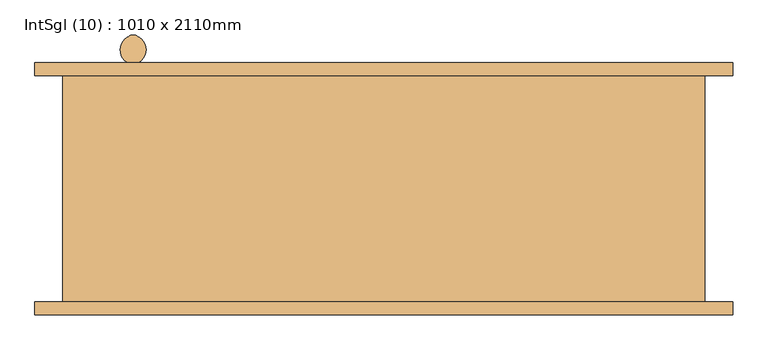
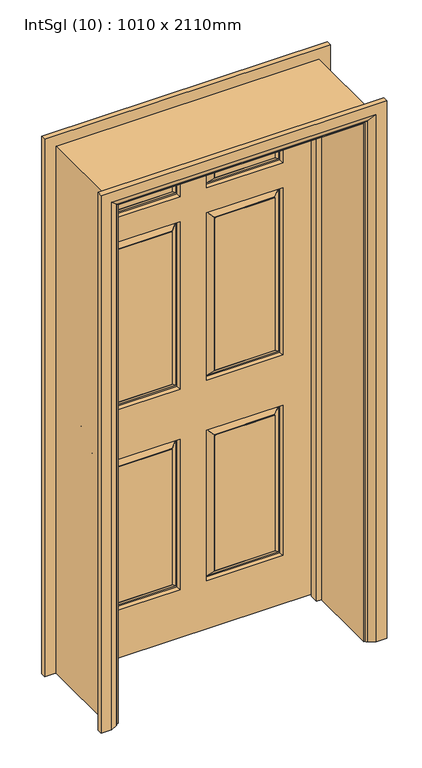
"""IFC4 building model written with IfcOpenShell, lengths in millimetres: door geometry, IntSgl (10) : 1010 x 2110mm."""

import ifcopenshell
import ifcopenshell.guid

model = None  # the IFC model being written
_history = None  # IfcOwnerHistory: only IFC2X3 demands one
_inside = {}  # id of a spatial element -> (the spatial element, [elements in it])
_under = {}  # id of a project, library or spatial element -> (it, [spatial elements below it])
_declared = {}  # id of a project -> (the project, [libraries it declares])
_typed = {}  # id of a type object -> (the type object, [elements of that type])
_made_of = {}  # id of a material, layer set ... -> (it, [elements and type objects made of it])


def new_model(schema):
    """Start an empty IFC model of exactly this schema.

    Asked for "IFC4X3", IfcOpenShell would pick the latest addendum, in which some entities
    have other attributes; the version numbers below select the first issue.
    IFC2X3 requires an IfcOwnerHistory on every rooted entity: one is made here for all.
    """
    global model, _history
    if schema == "IFC4X3":
        model = ifcopenshell.file(schema_version=(4, 3, 0, 0))
    else:
        model = ifcopenshell.file(schema=schema)
    _inside.clear()
    _under.clear()
    _declared.clear()
    _typed.clear()
    _made_of.clear()
    _history = None
    if model.schema == "IFC2X3":
        org = make("IfcOrganization", Name="unknown")
        user = make(
            "IfcPersonAndOrganization",
            ThePerson=make("IfcPerson", FamilyName="unknown"),
            TheOrganization=org,
        )
        app = make(
            "IfcApplication",
            ApplicationDeveloper=org,
            Version="unknown",
            ApplicationFullName="unknown",
            ApplicationIdentifier="unknown",
        )
        _history = make(
            "IfcOwnerHistory",
            OwningUser=user,
            OwningApplication=app,
            ChangeAction="ADDED",
            CreationDate=0,
        )
    return model


def make(cls, **values):
    """One entity of the class cls with the attributes given. An attribute that is None is left unset."""
    return model.create_entity(
        cls, **{name: value for name, value in values.items() if value is not None}
    )


def rooted(cls, **values):
    """An entity with a GlobalId (a new one), such as an element, a storey or a relation."""
    return make(cls, GlobalId=ifcopenshell.guid.new(), OwnerHistory=_history, **values)


def si_unit(unit_type, name, prefix=None):
    """IfcSIUnit, for example si_unit("LENGTHUNIT", "METRE", prefix="MILLI")."""
    return make("IfcSIUnit", UnitType=unit_type, Prefix=prefix, Name=name)


def assignment(units):
    """IfcUnitAssignment: the units of a project."""
    return None if units is None else make("IfcUnitAssignment", Units=units)


def point(xyz):
    """IfcCartesianPoint."""
    return None if xyz is None else make("IfcCartesianPoint", Coordinates=xyz)


def direction(xyz):
    """IfcDirection."""
    return None if xyz is None else make("IfcDirection", DirectionRatios=xyz)


def frame(location, z_axis=None, x_axis=None):
    """IfcAxis2Placement3D, a coordinate frame: its origin and axes. An axis left out is left unset."""
    return make(
        "IfcAxis2Placement3D",
        Location=point(location),
        Axis=direction(z_axis),
        RefDirection=direction(x_axis),
    )


def origin():
    """The frame at (0, 0, 0) with its axes left unset."""
    return frame((0.0, 0.0, 0.0))


def place(relative_to, where):
    """IfcLocalPlacement: puts the frame where relative to a parent placement (None: the world)."""
    return make(
        "IfcLocalPlacement", PlacementRelTo=relative_to, RelativePlacement=where
    )


def context(
    kind, dimensions, precision=None, world=None, true_north=None, identifier=None
):
    """IfcGeometricRepresentationContext, for example the 3D "Model" context."""
    return make(
        "IfcGeometricRepresentationContext",
        ContextIdentifier=identifier,
        ContextType=kind,
        CoordinateSpaceDimension=dimensions,
        Precision=precision,
        WorldCoordinateSystem=world,
        TrueNorth=true_north,
    )


def project(units=None, contexts=None):
    """IfcProject with its units and contexts."""
    return rooted(
        "IfcProject",
        Name="project",
        RepresentationContexts=contexts,
        UnitsInContext=assignment(units),
    )


def spatial(cls, under=None, at=None, **own):
    """A site, building, storey or space (cls), placed at a placement, below another one or the project."""
    s = rooted(cls, ObjectPlacement=at, **own)
    if under is not None:
        _under.setdefault(under.id(), (under, []))[1].append(s)
    return s


def polyline(points):
    """IfcPolyline through the points."""
    return make("IfcPolyline", Points=[point(p) for p in points])


def circle_curve(where, radius):
    """IfcCircle in the frame where."""
    return make("IfcCircle", Position=where, Radius=radius)


def ellipse_curve(where, semi_axis1, semi_axis2):
    """IfcEllipse in the frame where."""
    return make(
        "IfcEllipse", Position=where, SemiAxis1=semi_axis1, SemiAxis2=semi_axis2
    )


def trimmed(basis, trim1, trim2, sense, master):
    """IfcTrimmedCurve: the piece of a basis curve between two trims."""
    return make(
        "IfcTrimmedCurve",
        BasisCurve=basis,
        Trim1=trim1,
        Trim2=trim2,
        SenseAgreement=sense,
        MasterRepresentation=master,
    )


def outline(outer, holes=None, kind="AREA"):
    """IfcArbitraryClosedProfileDef: a profile drawn as a closed curve; with holes, ...WithVoids."""
    if holes is None:
        return make("IfcArbitraryClosedProfileDef", ProfileType=kind, OuterCurve=outer)
    return make(
        "IfcArbitraryProfileDefWithVoids",
        ProfileType=kind,
        OuterCurve=outer,
        InnerCurves=holes,
    )


def extrude(swept, where, along, depth):
    """IfcExtrudedAreaSolid: the profile swept, set in the frame where, extruded along a direction by depth."""
    return make(
        "IfcExtrudedAreaSolid",
        SweptArea=swept,
        Position=where,
        ExtrudedDirection=direction(along),
        Depth=depth,
    )


def faces_of(points, faces, orient=None, outer=None):
    """IfcFace entities. A face is a list of loops; a loop is a list of indices into points, from 0.

    orient and outer hold one flag for each loop. By default every Orientation is true, the
    first loop of a face is its IfcFaceOuterBound and the others are IfcFaceBound.
    """
    made = []
    for i, loops in enumerate(faces):
        bounds = []
        for j, loop in enumerate(loops):
            is_outer = j == 0 if outer is None else outer[i][j]
            bounds.append(
                make(
                    "IfcFaceOuterBound" if is_outer else "IfcFaceBound",
                    Bound=make("IfcPolyLoop", Polygon=[points[k] for k in loop]),
                    Orientation=True if orient is None else orient[i][j],
                )
            )
        made.append(make("IfcFace", Bounds=bounds))
    return made


def faceted_brep(points, faces, orient=None, outer=None, voids=None):
    """IfcFacetedBrep: a solid bounded by flat faces; with voids (closed shells), ...WithVoids."""
    shared = [point(p) for p in points]
    hull = make("IfcClosedShell", CfsFaces=faces_of(shared, faces, orient, outer))
    if voids is None:
        return make("IfcFacetedBrep", Outer=hull)
    return make(
        "IfcFacetedBrepWithVoids",
        Outer=hull,
        Voids=[
            make(cls, CfsFaces=faces_of(shared, fs, o, b)) for cls, fs, o, b in voids
        ],
    )


def shape(context_of_items, identifier, shape_type, items):
    """IfcShapeRepresentation: the items that make up one representation, for example the "Body"."""
    return make(
        "IfcShapeRepresentation",
        ContextOfItems=context_of_items,
        RepresentationIdentifier=identifier,
        RepresentationType=shape_type,
        Items=items,
    )


def source(mapping_origin, context_of_items, identifier, shape_type, items):
    """IfcRepresentationMap: a shape defined once, which mapped items show again and again."""
    return make(
        "IfcRepresentationMap",
        MappingOrigin=mapping_origin,
        MappedRepresentation=shape(context_of_items, identifier, shape_type, items),
    )


def transform(
    local_origin,
    x_axis=None,
    y_axis=None,
    z_axis=None,
    scale=None,
    scale2=None,
    scale3=None,
    uniform=True,
):
    """IfcCartesianTransformationOperator3D, or its non-uniform kind. x_axis, y_axis, z_axis: its Axis1, 2, 3."""
    if uniform:
        return make(
            "IfcCartesianTransformationOperator3D",
            Axis1=direction(x_axis),
            Axis2=direction(y_axis),
            LocalOrigin=point(local_origin),
            Scale=scale,
            Axis3=direction(z_axis),
        )
    return make(
        "IfcCartesianTransformationOperator3DnonUniform",
        Axis1=direction(x_axis),
        Axis2=direction(y_axis),
        LocalOrigin=point(local_origin),
        Scale=scale,
        Axis3=direction(z_axis),
        Scale2=scale2,
        Scale3=scale3,
    )


def mapped(mapping_source, mapping_target):
    """IfcMappedItem: shows the shape of a source again, moved by a transform."""
    return make(
        "IfcMappedItem", MappingSource=mapping_source, MappingTarget=mapping_target
    )


def made_of(thing, what):
    """Note that an element or type object is made of a material, layer set ...; save() writes the relation."""
    if what is not None:
        _made_of.setdefault(what.id(), (what, []))[1].append(thing)
    return thing


def element(
    cls,
    number,
    at=None,
    inside=None,
    cuts=None,
    type_object=None,
    material=None,
    context=None,
    identifier="Body",
    shape_type=None,
    held_by="IfcProductDefinitionShape",
    body=None,
    shapes=None,
    **own,
):
    """One element of the class cls, such as IfcWall. Its Tag is "e" and its number.

    at: its placement. inside: the storey or other place that contains it. cuts: it is an
    opening in that element (IfcRelVoidsElement). A single representation is given by context,
    identifier, shape_type and body (its items); several are given by shapes. held_by: the class
    of the entity that holds the representations. save() writes the other relations.
    """
    e = rooted(cls, Tag="e%d" % number, ObjectPlacement=at, **own)
    if body is not None:
        shapes = [shape(context, identifier, shape_type, body)]
    if shapes is not None:
        e.Representation = make(held_by, Representations=shapes)
    if inside is not None:
        _inside.setdefault(inside.id(), (inside, []))[1].append(e)
    if cuts is not None:
        rooted(
            "IfcRelVoidsElement", RelatingBuildingElement=cuts, RelatedOpeningElement=e
        )
    if type_object is not None:
        _typed.setdefault(type_object.id(), (type_object, []))[1].append(e)
    return made_of(e, material)


def aggregate(whole, parts):
    """IfcRelAggregates: a whole, such as a stair, and the parts it consists of."""
    return rooted("IfcRelAggregates", RelatingObject=whole, RelatedObjects=parts)


def save(model, path):
    """Write the relations noted so far, then the file.

    IfcRelAggregates (storeys below a building ...), IfcRelContainedInSpatialStructure (elements
    in a storey), IfcRelDefinesByType, IfcRelAssociatesMaterial and IfcRelDeclares: one each for
    every whole, place, type object, material and project.
    """
    for whole, parts in _under.values():
        aggregate(whole, parts)
    for where, things in _inside.values():
        rooted(
            "IfcRelContainedInSpatialStructure",
            RelatedElements=things,
            RelatingStructure=where,
        )
    for kind, things in _typed.values():
        rooted("IfcRelDefinesByType", RelatedObjects=things, RelatingType=kind)
    for what, things in _made_of.values():
        rooted("IfcRelAssociatesMaterial", RelatedObjects=things, RelatingMaterial=what)
    for by, libraries in _declared.values():
        rooted("IfcRelDeclares", RelatingContext=by, RelatedDefinitions=libraries)
    model.write(path)


def plane_surface(at):
    """IfcPlane: the flat surface through the origin of the frame at, square to its z axis."""
    return make("IfcPlane", Position=at)


def cylinder_surface(at, radius):
    """IfcCylindricalSurface: all points at the distance radius from the z axis of the frame at."""
    return make("IfcCylindricalSurface", Position=at, Radius=radius)


def revolved_surface(curve, axis_point, axis_direction):
    """IfcSurfaceOfRevolution: the curve turned about the line through axis_point along axis_direction."""
    return make(
        "IfcSurfaceOfRevolution",
        SweptCurve=make("IfcArbitraryOpenProfileDef", ProfileType="CURVE", Curve=curve),
        AxisPosition=make("IfcAxis1Placement", Location=point(axis_point), Axis=direction(axis_direction)),
    )


def advanced_brep(points, edges, surfaces, faces):
    """IfcAdvancedBrep: a solid bounded by faces that lie on surfaces and meet in shared edges.

    An edge is (start, end): straight between two places in points (the first is 0);
    or (start, end, curve); or (start, end, curve, False) where it runs against its curve.
    A face is (place in surfaces, loops), or (place, loops, False) where it looks against
    its surface's normal. A loop lists edges by number (the first is 1), with a minus sign
    where the edge is run from its end to its start. The first loop is the outer one.
    """
    corners = [point(p) for p in points]
    vertices = [make("IfcVertexPoint", VertexGeometry=c) for c in corners]
    made = []
    for start, end, *more in edges:
        made.append(
            make(
                "IfcEdgeCurve",
                EdgeStart=vertices[start],
                EdgeEnd=vertices[end],
                EdgeGeometry=more[0] if more else make("IfcPolyline", Points=[corners[start], corners[end]]),
                SameSense=more[1] if len(more) > 1 else True,
            )
        )
    hull = []
    for where, loops, *sense in faces:
        bounds = []
        for j, loop in enumerate(loops):
            ring = [make("IfcOrientedEdge", EdgeElement=made[abs(k) - 1], Orientation=k > 0) for k in loop]
            bounds.append(
                make(
                    "IfcFaceOuterBound" if j == 0 else "IfcFaceBound",
                    Bound=make("IfcEdgeLoop", EdgeList=ring),
                    Orientation=True,
                )
            )
        hull.append(make("IfcAdvancedFace", Bounds=bounds, FaceSurface=surfaces[where], SameSense=sense[0] if sense else True))
    return make("IfcAdvancedBrep", Outer=make("IfcClosedShell", CfsFaces=hull))


def intsgl_10_1010_x_2110mm_e5549126(model_context):
    return source(origin(), model_context, "Body", "SolidModel", [
        advanced_brep(
        [(-383.0, 118.0, 900.0), (-388.0, 73.562589, 900.0), (-393.0, 118.0, 900.0), (-393.0, 133.0, 900.0), (-383.0, 133.0, 900.0), (-408.0, 137.0, 900.0), (-368.0, 137.0, 900.0), (-408.0, 133.0, 900.0), (-368.0, 133.0, 900.0)],
        [
            (0, 1, circle_curve(frame((-391.1884862, 96.4213505, 900.0), z_axis=(0.0, 0.0, -1.0), x_axis=(0.0, 1.0, 0.0)), 23.0800654)),
            (1, 2, circle_curve(frame((-384.8115138, 96.4213505, 900.0), z_axis=(0.0, 0.0, -1.0), x_axis=(0.0, 1.0, 0.0)), 23.0800654)),
            (2, 0, circle_curve(frame((-388.0, 118.0, 900.0), z_axis=(0.0, -1.0, 0.0), x_axis=(-1.0, 0.0, 0.0)), 5.0)),
            (0, 2, circle_curve(frame((-388.0, 118.0, 900.0), z_axis=(0.0, -1.0, 0.0), x_axis=(-1.0, 0.0, 0.0)), 5.0)),
            (2, 3),
            (3, 4, circle_curve(frame((-388.0, 133.0, 900.0), z_axis=(0.0, -1.0, 0.0), x_axis=(-1.0, 0.0, 0.0)), 5.0)),
            (4, 0),
            (4, 3, circle_curve(frame((-388.0, 133.0, 900.0), z_axis=(0.0, -1.0, 0.0), x_axis=(-1.0, 0.0, 0.0)), 5.0)),
            (5, 6, circle_curve(frame((-388.0, 137.0, 900.0), z_axis=(0.0, 1.0, 0.0), x_axis=(1.0, 0.0, 0.0)), 20.0)),
            (6, 5, circle_curve(frame((-388.0, 137.0, 900.0), z_axis=(0.0, 1.0, 0.0), x_axis=(1.0, 0.0, 0.0)), 20.0)),
            (7, 8, circle_curve(frame((-388.0, 133.0, 900.0), z_axis=(0.0, -1.0, 0.0), x_axis=(1.0, 0.0, 0.0)), 20.0)),
            (8, 7, circle_curve(frame((-388.0, 133.0, 900.0), z_axis=(0.0, -1.0, 0.0), x_axis=(1.0, 0.0, 0.0)), 20.0)),
            (6, 8),
            (7, 5),
        ],
        [
            revolved_surface(trimmed(ellipse_curve(frame((-384.8115138, 96.4213505, 900.0), z_axis=(0.0, 0.0, -1.0), x_axis=(0.0, 1.0, 0.0)), 23.0800654, 23.0800654), [point((-388.0, 73.562589, 900.0))], [point((-393.0, 118.0, 900.0))], True, "CARTESIAN"), (-388.0, 133.0, 900.0), (0.0, 1.0, 0.0)),
            cylinder_surface(frame((-388.0, 133.0, 900.0), z_axis=(0.0, 1.0, 0.0), x_axis=(-1.0, 0.0, 0.0)), 5.0),
            plane_surface(frame((-368.0, 137.0, 900.0), z_axis=(0.0, 1.0, 0.0), x_axis=(0.0, 0.0, 1.0))),
            plane_surface(frame((-368.0, 133.0, 900.0), z_axis=(0.0, -1.0, 0.0), x_axis=(0.0, 0.0, -1.0))),
            cylinder_surface(frame((-388.0, 133.0, 900.0), z_axis=(0.0, 1.0, 0.0), x_axis=(1.0, 0.0, 0.0)), 20.0),
        ],
        [
            (0, [[1, 2, 3]]),
            (0, [[-1, 4, -2]]),
            (1, [[5, 6, 7, -3]]),
            (1, [[-7, 8, -5, -4]]),
            (2, [[9, 10]]),
            (3, [[11, 12], [-8, -6]]),
            (4, [[13, -11, 14, -10]]),
            (4, [[-14, -12, -13, -9]]),
        ],
    ),
        advanced_brep(
        [(-383.0, 194.0, 900.0), (-393.0, 194.0, 900.0), (-388.0, 238.437411, 900.0), (-383.0, 179.0, 900.0), (-393.0, 179.0, 900.0), (-408.0, 175.0, 900.0), (-368.0, 175.0, 900.0), (-408.0, 179.0, 900.0), (-368.0, 179.0, 900.0)],
        [
            (0, 1, circle_curve(frame((-388.0, 194.0, 900.0), z_axis=(0.0, 1.0, 0.0), x_axis=(-1.0, 0.0, 0.0)), 5.0)),
            (1, 2, circle_curve(frame((-384.8115138, 215.5786495, 900.0), z_axis=(0.0, 0.0, -1.0), x_axis=(0.0, -1.0, 0.0)), 23.0800654)),
            (2, 0, circle_curve(frame((-391.1884862, 215.5786495, 900.0), z_axis=(0.0, 0.0, -1.0), x_axis=(0.0, -1.0, 0.0)), 23.0800654)),
            (1, 0, circle_curve(frame((-388.0, 194.0, 900.0), z_axis=(0.0, 1.0, 0.0), x_axis=(-1.0, 0.0, 0.0)), 5.0)),
            (0, 3),
            (3, 4, circle_curve(frame((-388.0, 179.0, 900.0), z_axis=(0.0, 1.0, 0.0), x_axis=(-1.0, 0.0, 0.0)), 5.0)),
            (4, 1),
            (4, 3, circle_curve(frame((-388.0, 179.0, 900.0), z_axis=(0.0, 1.0, 0.0), x_axis=(-1.0, 0.0, 0.0)), 5.0)),
            (5, 6, circle_curve(frame((-388.0, 175.0, 900.0), z_axis=(0.0, -1.0, 0.0), x_axis=(1.0, 0.0, 0.0)), 20.0)),
            (6, 5, circle_curve(frame((-388.0, 175.0, 900.0), z_axis=(0.0, -1.0, 0.0), x_axis=(1.0, 0.0, 0.0)), 20.0)),
            (7, 8, circle_curve(frame((-388.0, 179.0, 900.0), z_axis=(0.0, 1.0, 0.0), x_axis=(1.0, 0.0, 0.0)), 20.0)),
            (8, 7, circle_curve(frame((-388.0, 179.0, 900.0), z_axis=(0.0, 1.0, 0.0), x_axis=(1.0, 0.0, 0.0)), 20.0)),
            (5, 7),
            (8, 6),
        ],
        [
            revolved_surface(trimmed(ellipse_curve(frame((-384.8115138, 215.5786495, 900.0), z_axis=(0.0, 0.0, 1.0), x_axis=(0.0, -1.0, 0.0)), 23.0800654, 23.0800654), [point((-388.0, 238.437411, 900.0))], [point((-393.0, 194.0, 900.0))], True, "CARTESIAN"), (-388.0, 179.0, 900.0), (0.0, -1.0, 0.0)),
            cylinder_surface(frame((-388.0, 179.0, 900.0), z_axis=(0.0, -1.0, 0.0), x_axis=(-1.0, 0.0, 0.0)), 5.0),
            plane_surface(frame((-368.0, 175.0, 900.0), z_axis=(0.0, -1.0, 0.0), x_axis=(0.0, 0.0, 1.0))),
            plane_surface(frame((-368.0, 179.0, 900.0), z_axis=(0.0, 1.0, 0.0), x_axis=(0.0, 0.0, -1.0))),
            cylinder_surface(frame((-388.0, 179.0, 900.0), z_axis=(0.0, -1.0, 0.0), x_axis=(1.0, 0.0, 0.0)), 20.0),
        ],
        [
            (0, [[1, 2, 3]]),
            (0, [[-2, 4, -3]]),
            (1, [[-1, 5, 6, 7]]),
            (1, [[-4, -7, 8, -5]]),
            (2, [[9, 10]]),
            (3, [[11, 12], [-6, -8]]),
            (4, [[-9, 13, -12, 14]]),
            (4, [[-10, -14, -11, -13]]),
        ],
    ),
        faceted_brep([(-463.0, 137.0, 2068.0), (-463.0, 137.0, 8.0), (463.0, 137.0, 8.0), (463.0, 137.0, 2068.0), (-50.0, 137.0, 800.0), (-50.0, 137.0, 200.0), (-338.0, 137.0, 200.0), (-338.0, 137.0, 800.0), (338.0, 137.0, 800.0), (338.0, 137.0, 200.0), (50.0, 137.0, 200.0), (50.0, 137.0, 800.0), (-50.0, 137.0, 1668.0), (-50.0, 137.0, 1000.0), (-338.0, 137.0, 1000.0), (-338.0, 137.0, 1668.0), (338.0, 137.0, 1668.0), (338.0, 137.0, 1000.0), (50.0, 137.0, 1000.0), (50.0, 137.0, 1668.0), (-50.0, 137.0, 1943.0), (-50.0, 137.0, 1768.0), (-338.0, 137.0, 1768.0), (-338.0, 137.0, 1943.0), (338.0, 137.0, 1943.0), (338.0, 137.0, 1768.0), (50.0, 137.0, 1768.0), (50.0, 137.0, 1943.0), (-80.0, 137.0, 230.0), (-80.0, 137.0, 770.0), (-308.0, 137.0, 770.0), (-308.0, 137.0, 230.0), (308.0, 137.0, 230.0), (308.0, 137.0, 770.0), (80.0, 137.0, 770.0), (80.0, 137.0, 230.0), (-80.0, 137.0, 1030.0), (-80.0, 137.0, 1638.0), (-308.0, 137.0, 1638.0), (-308.0, 137.0, 1030.0), (308.0, 137.0, 1030.0), (308.0, 137.0, 1638.0), (80.0, 137.0, 1638.0), (80.0, 137.0, 1030.0), (-80.0, 137.0, 1798.0), (-80.0, 137.0, 1913.0), (-308.0, 137.0, 1913.0), (-308.0, 137.0, 1798.0), (308.0, 137.0, 1798.0), (308.0, 137.0, 1913.0), (80.0, 137.0, 1913.0), (80.0, 137.0, 1798.0), (-463.0, 175.0, 2068.0), (463.0, 175.0, 2068.0), (463.0, 175.0, 8.0), (-463.0, 175.0, 8.0), (50.0, 175.0, 800.0), (50.0, 175.0, 200.0), (338.0, 175.0, 200.0), (338.0, 175.0, 800.0), (-338.0, 175.0, 800.0), (-338.0, 175.0, 200.0), (-50.0, 175.0, 200.0), (-50.0, 175.0, 800.0), (50.0, 175.0, 1668.0), (50.0, 175.0, 1000.0), (338.0, 175.0, 1000.0), (338.0, 175.0, 1668.0), (-338.0, 175.0, 1668.0), (-338.0, 175.0, 1000.0), (-50.0, 175.0, 1000.0), (-50.0, 175.0, 1668.0), (50.0, 175.0, 1943.0), (50.0, 175.0, 1768.0), (338.0, 175.0, 1768.0), (338.0, 175.0, 1943.0), (-338.0, 175.0, 1943.0), (-338.0, 175.0, 1768.0), (-50.0, 175.0, 1768.0), (-50.0, 175.0, 1943.0), (80.0, 175.0, 230.0), (80.0, 175.0, 770.0), (308.0, 175.0, 770.0), (308.0, 175.0, 230.0), (-308.0, 175.0, 230.0), (-308.0, 175.0, 770.0), (-80.0, 175.0, 770.0), (-80.0, 175.0, 230.0), (80.0, 175.0, 1030.0), (80.0, 175.0, 1638.0), (308.0, 175.0, 1638.0), (308.0, 175.0, 1030.0), (-308.0, 175.0, 1030.0), (-308.0, 175.0, 1638.0), (-80.0, 175.0, 1638.0), (-80.0, 175.0, 1030.0), (80.0, 175.0, 1798.0), (80.0, 175.0, 1913.0), (308.0, 175.0, 1913.0), (308.0, 175.0, 1798.0), (-308.0, 175.0, 1798.0), (-308.0, 175.0, 1913.0), (-80.0, 175.0, 1913.0), (-80.0, 175.0, 1798.0), (80.0, 174.0, 230.0), (80.0, 174.0, 770.0), (58.0, 160.0, 208.0), (58.0, 160.0, 792.0), (78.0, 174.0, 772.0), (78.0, 174.0, 228.0), (53.0, 160.0, 797.0), (53.0, 160.0, 203.0), (308.0, 174.0, 770.0), (330.0, 160.0, 792.0), (310.0, 174.0, 772.0), (335.0, 160.0, 797.0), (308.0, 174.0, 230.0), (330.0, 160.0, 208.0), (310.0, 174.0, 228.0), (335.0, 160.0, 203.0), (-308.0, 174.0, 230.0), (-308.0, 174.0, 770.0), (-330.0, 160.0, 208.0), (-330.0, 160.0, 792.0), (-310.0, 174.0, 772.0), (-310.0, 174.0, 228.0), (-335.0, 160.0, 797.0), (-335.0, 160.0, 203.0), (-80.0, 174.0, 770.0), (-58.0, 160.0, 792.0), (-78.0, 174.0, 772.0), (-53.0, 160.0, 797.0), (-80.0, 174.0, 230.0), (-58.0, 160.0, 208.0), (-78.0, 174.0, 228.0), (-53.0, 160.0, 203.0), (80.0, 174.0, 1030.0), (80.0, 174.0, 1638.0), (58.0, 160.0, 1008.0), (58.0, 160.0, 1660.0), (78.0, 174.0, 1640.0), (78.0, 174.0, 1028.0), (53.0, 160.0, 1665.0), (53.0, 160.0, 1003.0), (308.0, 174.0, 1638.0), (330.0, 160.0, 1660.0), (310.0, 174.0, 1640.0), (335.0, 160.0, 1665.0), (308.0, 174.0, 1030.0), (330.0, 160.0, 1008.0), (310.0, 174.0, 1028.0), (335.0, 160.0, 1003.0), (-308.0, 174.0, 1030.0), (-308.0, 174.0, 1638.0), (-330.0, 160.0, 1008.0), (-330.0, 160.0, 1660.0), (-310.0, 174.0, 1640.0), (-310.0, 174.0, 1028.0), (-335.0, 160.0, 1665.0), (-335.0, 160.0, 1003.0), (-80.0, 174.0, 1638.0), (-58.0, 160.0, 1660.0), (-78.0, 174.0, 1640.0), (-53.0, 160.0, 1665.0), (-80.0, 174.0, 1030.0), (-58.0, 160.0, 1008.0), (-78.0, 174.0, 1028.0), (-53.0, 160.0, 1003.0), (80.0, 174.0, 1798.0), (80.0, 174.0, 1913.0), (58.0, 160.0, 1776.0), (58.0, 160.0, 1935.0), (78.0, 174.0, 1915.0), (78.0, 174.0, 1796.0), (53.0, 160.0, 1940.0), (53.0, 160.0, 1771.0), (308.0, 174.0, 1913.0), (330.0, 160.0, 1935.0), (310.0, 174.0, 1915.0), (335.0, 160.0, 1940.0), (308.0, 174.0, 1798.0), (330.0, 160.0, 1776.0), (310.0, 174.0, 1796.0), (335.0, 160.0, 1771.0), (-308.0, 174.0, 1798.0), (-308.0, 174.0, 1913.0), (-330.0, 160.0, 1776.0), (-330.0, 160.0, 1935.0), (-310.0, 174.0, 1915.0), (-310.0, 174.0, 1796.0), (-335.0, 160.0, 1940.0), (-335.0, 160.0, 1771.0), (-80.0, 174.0, 1913.0), (-58.0, 160.0, 1935.0), (-78.0, 174.0, 1915.0), (-53.0, 160.0, 1940.0), (-80.0, 174.0, 1798.0), (-58.0, 160.0, 1776.0), (-78.0, 174.0, 1796.0), (-53.0, 160.0, 1771.0), (-80.0, 138.0, 230.0), (-80.0, 138.0, 770.0), (-58.0, 152.0, 208.0), (-58.0, 152.0, 792.0), (-78.0, 138.0, 772.0), (-78.0, 138.0, 228.0), (-53.0, 152.0, 797.0), (-53.0, 152.0, 203.0), (-308.0, 138.0, 770.0), (-330.0, 152.0, 792.0), (-310.0, 138.0, 772.0), (-335.0, 152.0, 797.0), (-308.0, 138.0, 230.0), (-330.0, 152.0, 208.0), (-310.0, 138.0, 228.0), (-335.0, 152.0, 203.0), (308.0, 138.0, 230.0), (308.0, 138.0, 770.0), (330.0, 152.0, 208.0), (330.0, 152.0, 792.0), (310.0, 138.0, 772.0), (310.0, 138.0, 228.0), (335.0, 152.0, 797.0), (335.0, 152.0, 203.0), (80.0, 138.0, 770.0), (58.0, 152.0, 792.0), (78.0, 138.0, 772.0), (53.0, 152.0, 797.0), (80.0, 138.0, 230.0), (58.0, 152.0, 208.0), (78.0, 138.0, 228.0), (53.0, 152.0, 203.0), (-80.0, 138.0, 1030.0), (-80.0, 138.0, 1638.0), (-58.0, 152.0, 1008.0), (-58.0, 152.0, 1660.0), (-78.0, 138.0, 1640.0), (-78.0, 138.0, 1028.0), (-53.0, 152.0, 1665.0), (-53.0, 152.0, 1003.0), (-308.0, 138.0, 1638.0), (-330.0, 152.0, 1660.0), (-310.0, 138.0, 1640.0), (-335.0, 152.0, 1665.0), (-308.0, 138.0, 1030.0), (-330.0, 152.0, 1008.0), (-310.0, 138.0, 1028.0), (-335.0, 152.0, 1003.0), (308.0, 138.0, 1030.0), (308.0, 138.0, 1638.0), (330.0, 152.0, 1008.0), (330.0, 152.0, 1660.0), (310.0, 138.0, 1640.0), (310.0, 138.0, 1028.0), (335.0, 152.0, 1665.0), (335.0, 152.0, 1003.0), (80.0, 138.0, 1638.0), (58.0, 152.0, 1660.0), (78.0, 138.0, 1640.0), (53.0, 152.0, 1665.0), (80.0, 138.0, 1030.0), (58.0, 152.0, 1008.0), (78.0, 138.0, 1028.0), (53.0, 152.0, 1003.0), (-80.0, 138.0, 1798.0), (-80.0, 138.0, 1913.0), (-58.0, 152.0, 1776.0), (-58.0, 152.0, 1935.0), (-78.0, 138.0, 1915.0), (-78.0, 138.0, 1796.0), (-53.0, 152.0, 1940.0), (-53.0, 152.0, 1771.0), (-308.0, 138.0, 1913.0), (-330.0, 152.0, 1935.0), (-310.0, 138.0, 1915.0), (-335.0, 152.0, 1940.0), (-308.0, 138.0, 1798.0), (-330.0, 152.0, 1776.0), (-310.0, 138.0, 1796.0), (-335.0, 152.0, 1771.0), (308.0, 138.0, 1798.0), (308.0, 138.0, 1913.0), (330.0, 152.0, 1776.0), (330.0, 152.0, 1935.0), (310.0, 138.0, 1915.0), (310.0, 138.0, 1796.0), (335.0, 152.0, 1940.0), (335.0, 152.0, 1771.0), (80.0, 138.0, 1913.0), (58.0, 152.0, 1935.0), (78.0, 138.0, 1915.0), (53.0, 152.0, 1940.0), (80.0, 138.0, 1798.0), (58.0, 152.0, 1776.0), (78.0, 138.0, 1796.0), (53.0, 152.0, 1771.0)], [[[0, 1, 2, 3], [4, 5, 6, 7], [8, 9, 10, 11], [12, 13, 14, 15], [16, 17, 18, 19], [20, 21, 22, 23], [24, 25, 26, 27]], [[28, 29, 30, 31]], [[32, 33, 34, 35]], [[36, 37, 38, 39]], [[40, 41, 42, 43]], [[44, 45, 46, 47]], [[48, 49, 50, 51]], [[52, 53, 54, 55], [56, 57, 58, 59], [60, 61, 62, 63], [64, 65, 66, 67], [68, 69, 70, 71], [72, 73, 74, 75], [76, 77, 78, 79]], [[80, 81, 82, 83]], [[84, 85, 86, 87]], [[88, 89, 90, 91]], [[92, 93, 94, 95]], [[96, 97, 98, 99]], [[100, 101, 102, 103]], [[1, 0, 52, 55]], [[2, 1, 55, 54]], [[3, 2, 54, 53]], [[0, 3, 53, 52]], [[104, 105, 81, 80]], [[106, 107, 108, 109]], [[56, 110, 111, 57]], [[81, 105, 112, 82]], [[108, 107, 113, 114]], [[110, 56, 59, 115]], [[82, 112, 116, 83]], [[114, 113, 117, 118]], [[115, 59, 58, 119]], [[104, 80, 83, 116]], [[109, 108, 114, 118], [105, 104, 116, 112]], [[106, 109, 118, 117]], [[111, 110, 115, 119], [107, 106, 117, 113]], [[57, 111, 119, 58]], [[120, 121, 85, 84]], [[122, 123, 124, 125]], [[60, 126, 127, 61]], [[85, 121, 128, 86]], [[124, 123, 129, 130]], [[126, 60, 63, 131]], [[86, 128, 132, 87]], [[130, 129, 133, 134]], [[131, 63, 62, 135]], [[120, 84, 87, 132]], [[125, 124, 130, 134], [121, 120, 132, 128]], [[122, 125, 134, 133]], [[127, 126, 131, 135], [123, 122, 133, 129]], [[61, 127, 135, 62]], [[136, 137, 89, 88]], [[138, 139, 140, 141]], [[64, 142, 143, 65]], [[89, 137, 144, 90]], [[140, 139, 145, 146]], [[142, 64, 67, 147]], [[90, 144, 148, 91]], [[146, 145, 149, 150]], [[147, 67, 66, 151]], [[136, 88, 91, 148]], [[141, 140, 146, 150], [137, 136, 148, 144]], [[138, 141, 150, 149]], [[143, 142, 147, 151], [139, 138, 149, 145]], [[65, 143, 151, 66]], [[152, 153, 93, 92]], [[154, 155, 156, 157]], [[68, 158, 159, 69]], [[93, 153, 160, 94]], [[156, 155, 161, 162]], [[158, 68, 71, 163]], [[94, 160, 164, 95]], [[162, 161, 165, 166]], [[163, 71, 70, 167]], [[152, 92, 95, 164]], [[157, 156, 162, 166], [153, 152, 164, 160]], [[154, 157, 166, 165]], [[159, 158, 163, 167], [155, 154, 165, 161]], [[69, 159, 167, 70]], [[168, 169, 97, 96]], [[170, 171, 172, 173]], [[72, 174, 175, 73]], [[97, 169, 176, 98]], [[172, 171, 177, 178]], [[174, 72, 75, 179]], [[98, 176, 180, 99]], [[178, 177, 181, 182]], [[179, 75, 74, 183]], [[168, 96, 99, 180]], [[173, 172, 178, 182], [169, 168, 180, 176]], [[170, 173, 182, 181]], [[175, 174, 179, 183], [171, 170, 181, 177]], [[73, 175, 183, 74]], [[184, 185, 101, 100]], [[186, 187, 188, 189]], [[76, 190, 191, 77]], [[101, 185, 192, 102]], [[188, 187, 193, 194]], [[190, 76, 79, 195]], [[102, 192, 196, 103]], [[194, 193, 197, 198]], [[195, 79, 78, 199]], [[184, 100, 103, 196]], [[189, 188, 194, 198], [185, 184, 196, 192]], [[186, 189, 198, 197]], [[191, 190, 195, 199], [187, 186, 197, 193]], [[77, 191, 199, 78]], [[200, 201, 29, 28]], [[202, 203, 204, 205]], [[4, 206, 207, 5]], [[29, 201, 208, 30]], [[204, 203, 209, 210]], [[206, 4, 7, 211]], [[30, 208, 212, 31]], [[210, 209, 213, 214]], [[211, 7, 6, 215]], [[200, 28, 31, 212]], [[205, 204, 210, 214], [201, 200, 212, 208]], [[202, 205, 214, 213]], [[207, 206, 211, 215], [203, 202, 213, 209]], [[5, 207, 215, 6]], [[216, 217, 33, 32]], [[218, 219, 220, 221]], [[8, 222, 223, 9]], [[33, 217, 224, 34]], [[220, 219, 225, 226]], [[222, 8, 11, 227]], [[34, 224, 228, 35]], [[226, 225, 229, 230]], [[227, 11, 10, 231]], [[216, 32, 35, 228]], [[221, 220, 226, 230], [217, 216, 228, 224]], [[218, 221, 230, 229]], [[223, 222, 227, 231], [219, 218, 229, 225]], [[9, 223, 231, 10]], [[232, 233, 37, 36]], [[234, 235, 236, 237]], [[12, 238, 239, 13]], [[37, 233, 240, 38]], [[236, 235, 241, 242]], [[238, 12, 15, 243]], [[38, 240, 244, 39]], [[242, 241, 245, 246]], [[243, 15, 14, 247]], [[232, 36, 39, 244]], [[237, 236, 242, 246], [233, 232, 244, 240]], [[234, 237, 246, 245]], [[239, 238, 243, 247], [235, 234, 245, 241]], [[13, 239, 247, 14]], [[248, 249, 41, 40]], [[250, 251, 252, 253]], [[16, 254, 255, 17]], [[41, 249, 256, 42]], [[252, 251, 257, 258]], [[254, 16, 19, 259]], [[42, 256, 260, 43]], [[258, 257, 261, 262]], [[259, 19, 18, 263]], [[248, 40, 43, 260]], [[253, 252, 258, 262], [249, 248, 260, 256]], [[250, 253, 262, 261]], [[255, 254, 259, 263], [251, 250, 261, 257]], [[17, 255, 263, 18]], [[264, 265, 45, 44]], [[266, 267, 268, 269]], [[20, 270, 271, 21]], [[45, 265, 272, 46]], [[268, 267, 273, 274]], [[270, 20, 23, 275]], [[46, 272, 276, 47]], [[274, 273, 277, 278]], [[275, 23, 22, 279]], [[264, 44, 47, 276]], [[269, 268, 274, 278], [265, 264, 276, 272]], [[266, 269, 278, 277]], [[271, 270, 275, 279], [267, 266, 277, 273]], [[21, 271, 279, 22]], [[280, 281, 49, 48]], [[282, 283, 284, 285]], [[24, 286, 287, 25]], [[49, 281, 288, 50]], [[284, 283, 289, 290]], [[286, 24, 27, 291]], [[50, 288, 292, 51]], [[290, 289, 293, 294]], [[291, 27, 26, 295]], [[280, 48, 51, 292]], [[285, 284, 290, 294], [281, 280, 292, 288]], [[282, 285, 294, 293]], [[287, 286, 291, 295], [283, 282, 293, 289]], [[25, 287, 295, 26]]]),
        advanced_brep(
        [(540.0, 195.0, 0.0), (540.0, 175.0, 0.0), (470.0, 175.0, 0.0), (474.0, 181.0, 0.0), (500.0, 195.0, 0.0), (540.0, 195.0, 2145.0), (540.0, 175.0, 2145.0), (-540.0, 175.0, 2145.0), (-540.0, 175.0, 0.0), (-470.0, 175.0, 0.0), (-470.0, 175.0, 2075.0), (470.0, 175.0, 2075.0), (474.0, 181.0, 2079.0), (500.0, 195.0, 2105.0), (-500.0, 195.0, 2105.0), (-500.0, 195.0, 0.0), (-540.0, 195.0, 0.0), (-540.0, 195.0, 2145.0), (-474.0, 181.0, 0.0), (-474.0, 181.0, 2079.0)],
        [
            (0, 1),
            (1, 2),
            (2, 3, circle_curve(frame((478.0, 174.0, 0.0), z_axis=(0.0, 0.0, -1.0), x_axis=(1.0, 0.0, 0.0)), 8.0622577)),
            (3, 4),
            (4, 0),
            (0, 5),
            (5, 6),
            (6, 1),
            (6, 7),
            (7, 8),
            (8, 9),
            (9, 10),
            (10, 11),
            (11, 2),
            (11, 12, ellipse_curve(frame((478.0, 174.0, 2083.0), z_axis=(0.7071067811865475, 0.0, -0.7071067811865475), x_axis=(-0.7071067811865474, 0.0, -0.7071067811865476)), 11.4017543, 8.0622577)),
            (12, 3),
            (12, 13),
            (13, 4),
            (13, 14),
            (14, 15),
            (15, 16),
            (16, 17),
            (17, 5),
            (7, 17),
            (16, 8),
            (15, 18),
            (18, 9, circle_curve(frame((-478.0, 174.0, 0.0), z_axis=(0.0, 0.0, -1.0), x_axis=(-1.0, 0.0, 0.0)), 8.0622577)),
            (19, 10, ellipse_curve(frame((-478.0, 174.0, 2083.0), z_axis=(-0.7071067811865475, 0.0, -0.7071067811865475), x_axis=(-0.7071067811865474, 0.0, 0.7071067811865476)), 11.4017543, 8.0622577)),
            (18, 19),
            (14, 19),
            (19, 12),
        ],
        [
            plane_surface(frame((470.0, 175.0, 0.0), z_axis=(0.0, 0.0, -1.0), x_axis=(0.0, 1.0, 0.0))),
            plane_surface(frame((540.0, 195.0, 0.0), z_axis=(1.0, 0.0, 0.0), x_axis=(0.0, 0.0, 1.0))),
            plane_surface(frame((540.0, 175.0, 0.0), z_axis=(0.0, -1.0, 0.0), x_axis=(0.0, 0.0, 1.0))),
            cylinder_surface(frame((478.0, 174.0, 0.0), z_axis=(0.0, 0.0, -1.0), x_axis=(1.0, 0.0, 0.0)), 8.0622577),
            plane_surface(frame((474.0, 181.0, 0.0), z_axis=(-0.4740998230350183, 0.8804710999221749, 0.0), x_axis=(0.0, 0.0, 1.0))),
            plane_surface(frame((500.0, 195.0, 0.0), z_axis=(0.0, 1.0, 0.0), x_axis=(0.0, 0.0, 1.0))),
            plane_surface(frame((-540.0, 195.0, 2145.0), z_axis=(-1.0, 0.0, 0.0), x_axis=(0.0, 0.0, -1.0))),
            plane_surface(frame((-470.0, 175.0, 0.0), z_axis=(0.0, 0.0, -1.0), x_axis=(0.0, 1.0, 0.0))),
            cylinder_surface(frame((-478.0, 174.0, 2075.0), z_axis=(0.0, 0.0, 1.0), x_axis=(-1.0, 0.0, 0.0)), 8.0622577),
            plane_surface(frame((-474.0, 181.0, 2079.0), z_axis=(0.4740998230350183, 0.8804710999221749, 0.0), x_axis=(0.0, 0.0, -1.0))),
            plane_surface(frame((540.0, 195.0, 2145.0), z_axis=(0.0, 0.0, 1.0), x_axis=(-1.0, 0.0, 0.0))),
            cylinder_surface(frame((470.0, 174.0, 2083.0), z_axis=(1.0, 0.0, 0.0), x_axis=(0.0, 0.0, 1.0)), 8.0622577),
            plane_surface(frame((474.0, 181.0, 2079.0), z_axis=(0.0, 0.8804710999221749, -0.4740998230350183), x_axis=(-1.0, 0.0, 0.0))),
        ],
        [
            (0, [[1, 2, 3, 4, 5]]),
            (1, [[-1, 6, 7, 8]]),
            (2, [[-2, -8, 9, 10, 11, 12, 13, 14]]),
            (3, [[-3, -14, 15, 16]]),
            (4, [[-4, -16, 17, 18]]),
            (5, [[-5, -18, 19, 20, 21, 22, 23, -6]]),
            (6, [[24, -22, 25, -10]]),
            (7, [[-21, 26, 27, -11, -25]]),
            (8, [[28, -12, -27, 29]]),
            (9, [[30, -29, -26, -20]]),
            (10, [[-7, -23, -24, -9]]),
            (11, [[-15, -13, -28, 31]]),
            (12, [[-17, -31, -30, -19]]),
        ],
    ),
        advanced_brep(
        [(-540.0, -195.0, 0.0), (-540.0, -175.0, 0.0), (-470.0, -175.0, 0.0), (-474.0, -181.0, 0.0), (-500.0, -195.0, 0.0), (-540.0, -195.0, 2145.0), (-540.0, -175.0, 2145.0), (540.0, -175.0, 2145.0), (540.0, -175.0, 0.0), (470.0, -175.0, 0.0), (470.0, -175.0, 2075.0), (-470.0, -175.0, 2075.0), (-474.0, -181.0, 2079.0), (-500.0, -195.0, 2105.0), (500.0, -195.0, 2105.0), (500.0, -195.0, 0.0), (540.0, -195.0, 0.0), (540.0, -195.0, 2145.0), (474.0, -181.0, 0.0), (474.0, -181.0, 2079.0)],
        [
            (0, 1),
            (1, 2),
            (2, 3, circle_curve(frame((-478.0, -174.0, 0.0), z_axis=(0.0, 0.0, -1.0), x_axis=(-1.0, 0.0, 0.0)), 8.0622577)),
            (3, 4),
            (4, 0),
            (0, 5),
            (5, 6),
            (6, 1),
            (6, 7),
            (7, 8),
            (8, 9),
            (9, 10),
            (10, 11),
            (11, 2),
            (11, 12, ellipse_curve(frame((-478.0, -174.0, 2083.0), z_axis=(-0.7071067811865475, 0.0, -0.7071067811865475), x_axis=(0.7071067811865474, 0.0, -0.7071067811865476)), 11.4017543, 8.0622577)),
            (12, 3),
            (12, 13),
            (13, 4),
            (13, 14),
            (14, 15),
            (15, 16),
            (16, 17),
            (17, 5),
            (7, 17),
            (16, 8),
            (15, 18),
            (18, 9, circle_curve(frame((478.0, -174.0, 0.0), z_axis=(0.0, 0.0, -1.0), x_axis=(1.0, 0.0, 0.0)), 8.0622577)),
            (19, 10, ellipse_curve(frame((478.0, -174.0, 2083.0), z_axis=(0.7071067811865475, 0.0, -0.7071067811865475), x_axis=(0.7071067811865474, 0.0, 0.7071067811865476)), 11.4017543, 8.0622577)),
            (18, 19),
            (14, 19),
            (19, 12),
        ],
        [
            plane_surface(frame((-470.0, -175.0, 0.0), z_axis=(0.0, 0.0, -1.0), x_axis=(0.0, -1.0, 0.0))),
            plane_surface(frame((-540.0, -195.0, 0.0), z_axis=(-1.0, 0.0, 0.0), x_axis=(0.0, 0.0, 1.0))),
            plane_surface(frame((-540.0, -175.0, 0.0), z_axis=(0.0, 1.0, 0.0), x_axis=(0.0, 0.0, 1.0))),
            cylinder_surface(frame((-478.0, -174.0, 0.0), z_axis=(0.0, 0.0, -1.0), x_axis=(-1.0, 0.0, 0.0)), 8.0622577),
            plane_surface(frame((-474.0, -181.0, 0.0), z_axis=(0.4740998230350183, -0.8804710999221749, 0.0), x_axis=(0.0, 0.0, 1.0))),
            plane_surface(frame((-500.0, -195.0, 0.0), z_axis=(0.0, -1.0, 0.0), x_axis=(0.0, 0.0, 1.0))),
            plane_surface(frame((540.0, -195.0, 2145.0), z_axis=(1.0, 0.0, 0.0), x_axis=(0.0, 0.0, -1.0))),
            plane_surface(frame((470.0, -175.0, 0.0), z_axis=(0.0, 0.0, -1.0), x_axis=(0.0, -1.0, 0.0))),
            cylinder_surface(frame((478.0, -174.0, 2075.0), z_axis=(0.0, 0.0, 1.0), x_axis=(1.0, 0.0, 0.0)), 8.0622577),
            plane_surface(frame((474.0, -181.0, 2079.0), z_axis=(-0.4740998230350183, -0.8804710999221749, 0.0), x_axis=(0.0, 0.0, -1.0))),
            plane_surface(frame((-540.0, -195.0, 2145.0), z_axis=(0.0, 0.0, 1.0), x_axis=(1.0, 0.0, 0.0))),
            cylinder_surface(frame((-470.0, -174.0, 2083.0), z_axis=(-1.0, 0.0, 0.0), x_axis=(0.0, 0.0, 1.0)), 8.0622577),
            plane_surface(frame((-474.0, -181.0, 2079.0), z_axis=(0.0, -0.8804710999221749, -0.4740998230350183), x_axis=(1.0, 0.0, 0.0))),
        ],
        [
            (0, [[1, 2, 3, 4, 5]]),
            (1, [[-1, 6, 7, 8]]),
            (2, [[-2, -8, 9, 10, 11, 12, 13, 14]]),
            (3, [[-3, -14, 15, 16]]),
            (4, [[-4, -16, 17, 18]]),
            (5, [[-5, -18, 19, 20, 21, 22, 23, -6]]),
            (6, [[24, -22, 25, -10]]),
            (7, [[-21, 26, 27, -11, -25]]),
            (8, [[28, -12, -27, 29]]),
            (9, [[30, -29, -26, -20]]),
            (10, [[-7, -23, -24, -9]]),
            (11, [[-15, -13, -28, 31]]),
            (12, [[-17, -31, -30, -19]]),
        ],
    ),
        extrude(outline(polyline([(0.0, -465.0), (0.0, -446.0), (2051.0, -446.0), (2051.0, 446.0), (0.0, 446.0), (0.0, 465.0), (2070.0, 465.0), (2070.0, -465.0), (0.0, -465.0)])), frame((0.0, 103.0, 0.0), z_axis=(0.0, 1.0, 0.0), x_axis=(0.0, 0.0, 1.0)), (0.0, 0.0, 1.0), 32.0),
        faceted_brep([(-465.0, 175.0, 0.0), (-465.0, -175.0, 0.0), (-497.0, -175.0, 0.0), (-497.0, 175.0, 0.0), (-465.0, 175.0, 2070.0), (-465.0, -175.0, 2070.0), (-497.0, -175.0, 2102.0), (-497.0, 175.0, 2102.0), (465.0, 175.0, 0.0), (497.0, 175.0, 0.0), (497.0, -175.0, 0.0), (465.0, -175.0, 0.0), (465.0, 175.0, 2070.0), (497.0, 175.0, 2102.0), (497.0, -175.0, 2102.0), (465.0, -175.0, 2070.0)], [[[0, 1, 2, 3]], [[1, 0, 4, 5]], [[2, 1, 5, 6]], [[3, 2, 6, 7]], [[0, 3, 7, 4]], [[8, 9, 10, 11]], [[12, 13, 9, 8]], [[13, 14, 10, 9]], [[14, 15, 11, 10]], [[15, 12, 8, 11]], [[5, 4, 12, 15]], [[6, 5, 15, 14]], [[7, 6, 14, 13]], [[4, 7, 13, 12]]]),
    ])


if __name__ == "__main__":
    model = new_model("IFC4")
    model_context = context("Model", 3, world=origin())
    ifc_project = project(units=[si_unit("LENGTHUNIT", "METRE", prefix="MILLI")], contexts=[model_context])
    site = spatial("IfcSite", under=ifc_project)
    building = spatial("IfcBuilding", under=site)
    placement = place(None, origin())
    intsgl_10_1010_x_2110mm_shape = intsgl_10_1010_x_2110mm_e5549126(model_context)
    element("IfcDoor", 1, ObjectType="IntSgl (10) : 1010 x 2110mm", at=placement, inside=building, context=model_context, shape_type="MappedRepresentation", body=[
        mapped(intsgl_10_1010_x_2110mm_shape, transform((0.0, 0.0, 0.0), x_axis=(1.0, 0.0, 0.0), y_axis=(0.0, 1.0, 0.0), z_axis=(0.0, 0.0, 1.0))),
    ])
    save(model, "model.ifc")

# Revit data of these elements
# Type "IntSgl (10) : 1010 x 2110mm"
#   Type Mark = "10"
#   Type Comments = "Internal Single"
#   Operation = "SingleSwingRight"
#   Manufacturer = "Revit"
#   Keynote = "L20"
#   Description = "Internal Single Door"
#   UnderCut = 8 mm
#   Tolerance = 2 mm
#   Thickness = 38 mm
#   Structural Tolerance = 8 mm
#   StopDepth = 32 mm
#   Stop Thickness = 19 mm
#   Stile Top Rail = 125 mm
#   Stile Shutting = 125 mm
#   Stile Muntin Rail = 100 mm
#   Stile Lock Rail = 200 mm
#   Stile Intermediate/Frieze = 100 mm
#   Stile Hanging = 125 mm
#   Stile Bottom Rail = 200 mm
#   Rough Width = 1010 mm
#   Rough Height = 2110 mm
#   Height to Top Lock Rail = 1000 mm
#   Handle Z Distance = 900 mm
#   Handle X Distance = 75 mm
#   Frame Thickness = 32 mm
#   Door Panel Width = 926 mm
#   Height = 2110 mm
#   Width = 1010 mm
#   Door Panel Thickness = 38 mm
#   Door Panel Offset = 0 mm
#   Door Panel Height = 2060 mm
#   Architrave Setback = 5 mm
#   Vis - Ironmongery = yes
#   Material Ironmongery = Door - Handle
#   Material Frame = Door - Frame/Mullion
#   Material Door = Door - Panel
#   Material Architrave = Door - Architrave
#   Function = (empty or 0)
#   Wall Closure = (empty or 0)
# Element 1 (IfcDoor, "IntSgl (10) : 1010 x 2110mm")
#   Materials on its faces: "Door - Panel", "Door - Architrave", "Door - Frame/Mullion", "Door - Handle"
# Materials
#   "Door - Handle": class "Miscellaneous", colour RGB 247 247 247, transparency 0
#   "Door - Frame/Mullion": class "Wood", colour RGB 212 179 113, transparency 0
#   "Door - Panel": class "Wood", colour RGB 210 159 95, transparency 0
#   "Door - Architrave": class "Wood", colour RGB 154 90 5, transparency 0
